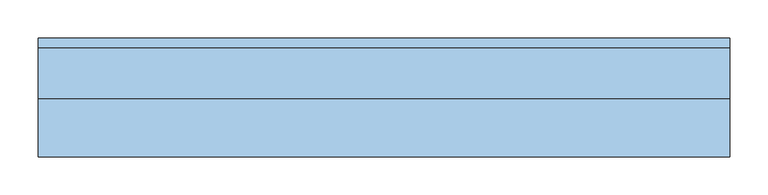
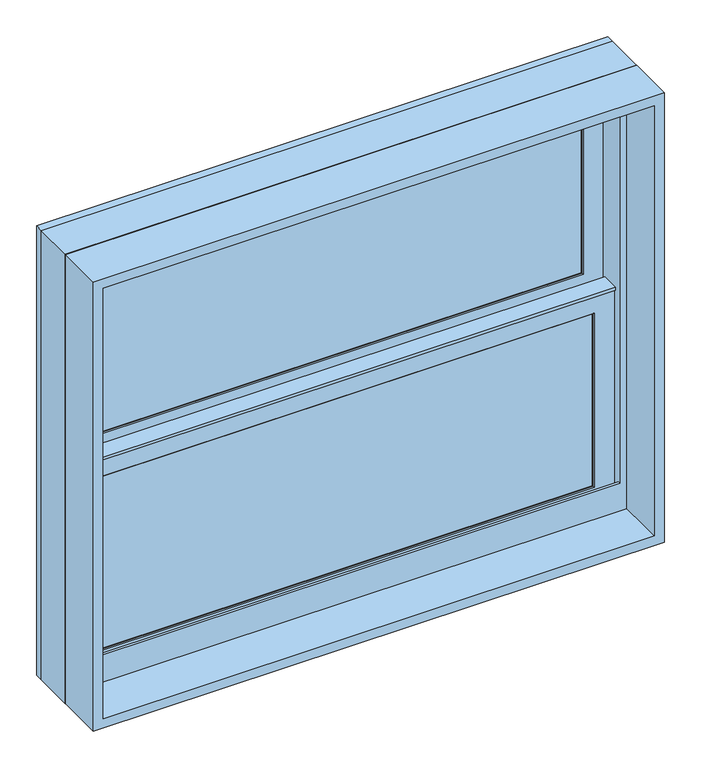
"""IFC4 building model written with IfcOpenShell, lengths in millimetres: window geometry, Window-Double_Hung-Marvin-Essential : ESDH3026."""

from ifc_helpers import new_model, si_unit, frame, origin, place, context, project, spatial, polyline, outline, extrude, faceted_brep, source, transform, mapped, element, save


def window_a7fb58c4(model_context):
    return source(origin(), model_context, "Body", "SolidModel", [
        extrude(outline(polyline([(140.7583333, 20.6375), (140.7583333, 15.875), (121.7083333, 15.875), (121.7083333, 20.6375), (140.7583333, 20.6375)])), frame((0.0, 0.0, 1746.25), z_axis=(0.0, 0.0, 1.0), x_axis=(1.0, 0.0, 0.0)), (0.0, 0.0, 1.0), 298.45),
        extrude(outline(polyline([(-121.7083333, 20.6375), (-121.7083333, 15.875), (-140.7583333, 15.875), (-140.7583333, 20.6375), (-121.7083333, 20.6375)])), frame((0.0, 0.0, 1746.25), z_axis=(0.0, 0.0, 1.0), x_axis=(1.0, 0.0, 0.0)), (0.0, 0.0, 1.0), 298.45),
        extrude(outline(polyline([(393.7, 20.6375), (393.7, 15.875), (-393.7, 15.875), (-393.7, 20.6375), (393.7, 20.6375)])), frame((0.0, 0.0, 1885.95), z_axis=(0.0, 0.0, 1.0), x_axis=(1.0, 0.0, 0.0)), (0.0, 0.0, 1.0), 19.05),
        extrude(outline(polyline([(-140.7583333, 46.83125), (-140.7583333, 51.59375), (-121.7083333, 51.59375), (-121.7083333, 46.83125), (-140.7583333, 46.83125)])), frame((0.0, 0.0, 2082.8), z_axis=(0.0, 0.0, 1.0), x_axis=(1.0, 0.0, 0.0)), (0.0, 0.0, 1.0), 298.45),
        extrude(outline(polyline([(121.7083333, 46.83125), (121.7083333, 51.59375), (140.7583333, 51.59375), (140.7583333, 46.83125), (121.7083333, 46.83125)])), frame((0.0, 0.0, 2082.8), z_axis=(0.0, 0.0, 1.0), x_axis=(1.0, 0.0, 0.0)), (0.0, 0.0, 1.0), 298.45),
        extrude(outline(polyline([(-393.7, 46.83125), (-393.7, 51.59375), (393.7, 51.59375), (393.7, 46.83125), (-393.7, 46.83125)])), frame((0.0, 0.0, 2222.5), z_axis=(0.0, 0.0, 1.0), x_axis=(1.0, 0.0, 0.0)), (0.0, 0.0, 1.0), 19.05),
        extrude(outline(polyline([(140.7583333, 20.6375), (121.7083333, 20.6375), (121.7083333, 25.4), (140.7583333, 25.4), (140.7583333, 20.6375)])), frame((0.0, 0.0, 1746.25), z_axis=(0.0, 0.0, 1.0), x_axis=(1.0, 0.0, 0.0)), (0.0, 0.0, 1.0), 298.45),
        extrude(outline(polyline([(-121.7083333, 20.6375), (-140.7583333, 20.6375), (-140.7583333, 25.4), (-121.7083333, 25.4), (-121.7083333, 20.6375)])), frame((0.0, 0.0, 1746.25), z_axis=(0.0, 0.0, 1.0), x_axis=(1.0, 0.0, 0.0)), (0.0, 0.0, 1.0), 298.45),
        extrude(outline(polyline([(393.7, 20.6375), (-393.7, 20.6375), (-393.7, 25.4), (393.7, 25.4), (393.7, 20.6375)])), frame((0.0, 0.0, 1885.95), z_axis=(0.0, 0.0, 1.0), x_axis=(1.0, 0.0, 0.0)), (0.0, 0.0, 1.0), 19.05),
        extrude(outline(polyline([(-140.7583333, 56.35625), (-121.7083333, 56.35625), (-121.7083333, 51.59375), (-140.7583333, 51.59375), (-140.7583333, 56.35625)])), frame((0.0, 0.0, 2082.8), z_axis=(0.0, 0.0, 1.0), x_axis=(1.0, 0.0, 0.0)), (0.0, 0.0, 1.0), 298.45),
        extrude(outline(polyline([(121.7083333, 56.35625), (140.7583333, 56.35625), (140.7583333, 51.59375), (121.7083333, 51.59375), (121.7083333, 56.35625)])), frame((0.0, 0.0, 2082.8), z_axis=(0.0, 0.0, 1.0), x_axis=(1.0, 0.0, 0.0)), (0.0, 0.0, 1.0), 298.45),
        extrude(outline(polyline([(-393.7, 56.35625), (393.7, 56.35625), (393.7, 51.59375), (-393.7, 51.59375), (-393.7, 56.35625)])), frame((0.0, 0.0, 2222.5), z_axis=(0.0, 0.0, 1.0), x_axis=(1.0, 0.0, 0.0)), (0.0, 0.0, 1.0), 19.05),
        faceted_brep([(-420.6875, 5.6780605, 2074.7351748), (-420.6875, 5.6780605, 2070.1), (420.6875, 5.6780605, 2070.1), (420.6875, 5.6780605, 2074.7351748), (-420.6875, 34.8118605, 2074.7351748), (420.6875, 34.8118605, 2074.7351748), (420.6875, 34.8118605, 2070.1), (-420.6875, 34.8118605, 2070.1), (-420.6875, 30.1625, 2070.1), (-420.6875, 30.1625, 1719.2625), (-420.6875, 8.9241104, 1719.2625), (-420.6875, 8.9241104, 2070.1), (420.6875, 8.9241104, 2070.1), (420.6875, 30.1625, 2070.1), (420.6875, 8.9241104, 1719.2625), (420.6875, 30.1625, 1719.2625), (-404.8034752, 11.90625, 2055.8034752), (-404.8034752, 30.1625, 2055.8034752), (404.8034752, 30.1625, 2055.8034752), (404.8034752, 11.90625, 2055.8034752), (-388.14375, 10.4662439, 2039.14375), (-388.14375, 11.90625, 2039.14375), (388.14375, 11.90625, 2039.14375), (388.14375, 10.4662439, 2039.14375), (389.6858834, 8.9241104, 2040.6858834), (-389.6858834, 8.9241104, 2040.6858834), (404.8034752, 30.1625, 1735.1465248), (404.8034752, 11.90625, 1735.1465248), (388.14375, 11.90625, 1751.80625), (388.14375, 10.4662439, 1751.80625), (389.6858834, 8.9241104, 1750.2641166), (-404.8034752, 30.1625, 1735.1465248), (-404.8034752, 11.90625, 1735.1465248), (-388.14375, 11.90625, 1751.80625), (-388.14375, 10.4662439, 1751.80625), (-389.6858834, 8.9241104, 1750.2641166)], [[[0, 1, 2, 3]], [[4, 5, 6, 7]], [[1, 0, 4, 7, 8, 9, 10, 11]], [[2, 1, 11, 12]], [[7, 6, 13, 8]], [[3, 2, 12, 14, 15, 13, 6, 5]], [[0, 3, 5, 4]], [[16, 17, 18, 19]], [[20, 21, 22, 23]], [[20, 23, 24, 25]], [[19, 18, 26, 27]], [[23, 22, 28, 29]], [[24, 23, 29, 30]], [[27, 26, 31, 32]], [[29, 28, 33, 34]], [[30, 29, 34, 35]], [[15, 14, 10, 9]], [[15, 9, 8, 13], [18, 17, 31, 26]], [[17, 16, 32, 31]], [[16, 19, 27, 32], [22, 21, 33, 28]], [[21, 20, 34, 33]], [[20, 25, 35, 34]], [[10, 14, 12, 11], [25, 24, 30, 35]]]),
        extrude(outline(polyline([(38.5955581, 2055.8125), (33.5778968, 2055.8125), (33.5778968, 2057.4), (39.9405976, 2057.4), (39.9405976, 2055.8125), (61.515625, 2055.8125), (47.6307501, 2052.4975159), (38.5955581, 2052.4975159), (38.5955581, 2055.8125)])), frame((-420.6875, 0.0, 0.0), z_axis=(1.0, 0.0, 0.0), x_axis=(0.0, 1.0, 0.0)), (0.0, 0.0, 1.0), 841.375),
        faceted_brep([(450.85, 0.0, 1689.1), (450.85, 0.0, 2438.4), (-450.85, 0.0, 2438.4), (-450.85, 0.0, 1689.1), (424.65625, 0.0, 1750.21875), (-424.65625, 0.0, 1750.21875), (-424.65625, 0.0, 2412.20625), (424.65625, 0.0, 2412.20625), (424.65625, 3.96875, 1689.1), (-424.65625, 3.96875, 1689.1), (-424.65625, 3.96875, 1750.21875), (424.65625, 3.96875, 1750.21875), (-450.85, 65.6828125, 1689.1), (-424.65625, 65.6828125, 1689.1), (424.65625, 65.6828125, 1689.1), (450.85, 65.6828125, 1689.1), (-450.85, 65.6828125, 2438.4), (450.85, 65.6828125, 2438.4), (424.65625, 65.6828125, 2412.20625), (-424.65625, 65.6828125, 2412.20625)], [[[0, 1, 2, 3], [4, 5, 6, 7]], [[8, 9, 10, 11]], [[5, 4, 11, 10]], [[0, 3, 12, 13, 9, 8, 14, 15]], [[13, 12, 16, 17, 15, 14, 18, 19]], [[13, 19, 6, 5, 10, 9]], [[7, 6, 19, 18]], [[18, 14, 8, 11, 4, 7]], [[1, 0, 15, 17]], [[2, 1, 17, 16]], [[3, 2, 16, 12]]]),
        faceted_brep([(424.65625, 30.1625, 2063.75), (423.06875, 30.1625, 2063.75), (423.06875, 30.1625, 1713.4544613), (424.65625, 30.1625, 1713.4544613), (-423.06875, 30.1625, 2063.75), (-424.65625, 30.1625, 2063.75), (-424.65625, 30.1625, 1713.4544613), (-423.06875, 30.1625, 1713.4544613), (423.06875, 63.5, 2063.75), (424.65625, 63.5, 2063.75), (424.65625, 63.5, 1706.9743077), (423.06875, 63.5, 1706.9743077), (-424.65625, 63.5, 2063.75), (-423.06875, 63.5, 2063.75), (-423.06875, 63.5, 1706.9743077), (-424.65625, 63.5, 1706.9743077), (435.9108932, 3.96875, 1718.5460105), (435.9108932, 3.96875, 1689.1), (435.9108932, 65.6828125, 1689.1), (435.9108932, 65.6828125, 1706.550012), (-435.9108932, 3.96875, 1689.1), (-435.9108932, 3.96875, 1718.5460105), (-435.9108932, 65.6828125, 1706.550012), (-435.9108932, 65.6828125, 1689.1), (435.9108932, 78.58125, 1704.0428097), (-435.9108932, 78.58125, 1704.0428097), (-433.8971252, 68.2348864, 1706.0539391), (-415.93135, 68.2348864, 1706.0539391), (-415.93135, 65.6828125, 1706.550012), (415.93135, 65.6828125, 1706.550012), (415.93135, 68.2348864, 1706.0539391), (433.8971252, 68.2348864, 1706.0539391), (-450.85, 65.6828125, 1689.1), (-450.85, 78.5948249, 1689.1), (450.85, 78.5948249, 1689.1), (450.85, 65.6828125, 1689.1), (-450.85, 78.58125, 2438.4), (450.85, 78.58125, 2438.4), (435.9108932, 78.58125, 2423.4608932), (-435.9108932, 78.58125, 2423.4608932), (-450.85, 65.6828125, 2438.4), (-433.8971252, 68.2348864, 2421.4471252), (433.8971252, 68.2348864, 2421.4471252), (415.93135, 68.2348864, 2403.48135), (-415.93135, 68.2348864, 2403.48135), (-415.93135, 65.6828125, 2403.48135), (415.93135, 65.6828125, 2403.48135), (450.85, 65.6828125, 2438.4)], [[[0, 1, 2, 3]], [[4, 5, 6, 7]], [[8, 9, 10, 11]], [[12, 13, 14, 15]], [[1, 8, 11, 2]], [[9, 0, 3, 10]], [[1, 0, 9, 8]], [[5, 4, 13, 12]], [[5, 12, 15, 6]], [[13, 4, 7, 14]], [[16, 17, 18, 19]], [[20, 21, 22, 23]], [[24, 25, 26, 27, 28, 22, 21, 16, 19, 29, 30, 31], [3, 2, 11, 10], [7, 6, 15, 14]], [[17, 16, 21, 20]], [[17, 20, 23, 32, 33, 34, 35, 18]], [[34, 33, 36, 37], [25, 24, 38, 39]], [[33, 32, 40, 36]], [[39, 41, 26, 25]], [[41, 42, 31, 30, 43, 44, 27, 26]], [[44, 45, 28, 27]], [[40, 32, 23, 22, 28, 45, 46, 29, 19, 18, 35, 47]], [[36, 40, 47, 37]], [[39, 38, 42, 41]], [[44, 43, 46, 45]], [[34, 37, 47, 35]], [[42, 38, 24, 31]], [[46, 43, 30, 29]]]),
        extrude(outline(polyline([(400.84375, 11.90625), (-400.84375, 11.90625), (-400.84375, 15.08125), (400.84375, 15.08125), (400.84375, 11.90625)])), frame((0.0, 0.0, 1739.10625), z_axis=(0.0, 0.0, 1.0), x_axis=(1.0, 0.0, 0.0)), (0.0, 0.0, 1.0), 312.7375),
        extrude(outline(polyline([(400.84375, 42.8625), (-400.84375, 42.8625), (-400.84375, 46.0375), (400.84375, 46.0375), (400.84375, 42.8625)])), frame((0.0, 0.0, 2075.65625), z_axis=(0.0, 0.0, 1.0), x_axis=(1.0, 0.0, 0.0)), (0.0, 0.0, 1.0), 312.7375),
        faceted_brep([(-388.14375, 31.194477, 2039.14375), (-389.6858834, 32.7366104, 2040.6858834), (389.6858834, 32.7366104, 2040.6858834), (388.14375, 31.194477, 2039.14375), (-388.14375, 30.1625, 2039.14375), (388.14375, 30.1625, 2039.14375), (-420.6875, 32.7366104, 2071.6875), (-420.6875, 30.1625, 2071.6875), (420.6875, 30.1625, 2071.6875), (420.6875, 32.7366104, 2071.6875), (389.6858834, 32.7366104, 1750.2641166), (388.14375, 31.194477, 1751.80625), (388.14375, 30.1625, 1751.80625), (420.6875, 30.1625, 1719.2625), (420.6875, 32.7366104, 1719.2625), (-389.6858834, 32.7366104, 1750.2641166), (-388.14375, 31.194477, 1751.80625), (-388.14375, 30.1625, 1751.80625), (-420.6875, 30.1625, 1719.2625), (-420.6875, 32.7366104, 1719.2625)], [[[0, 1, 2, 3]], [[4, 0, 3, 5]], [[6, 7, 8, 9]], [[3, 2, 10, 11]], [[5, 3, 11, 12]], [[9, 8, 13, 14]], [[11, 10, 15, 16]], [[12, 11, 16, 17]], [[14, 13, 18, 19]], [[9, 14, 19, 6], [1, 15, 10, 2]], [[16, 15, 1, 0]], [[17, 16, 0, 4]], [[7, 18, 13, 8], [5, 12, 17, 4]], [[19, 18, 7, 6]]]),
        faceted_brep([(-404.8034752, 42.8625, 2392.3534752), (-404.8034752, 61.11875, 2392.3534752), (404.8034752, 61.11875, 2392.3534752), (404.8034752, 42.8625, 2392.3534752), (-388.14375, 41.4224939, 2375.69375), (-388.14375, 42.8625, 2375.69375), (388.14375, 42.8625, 2375.69375), (388.14375, 41.4224939, 2375.69375), (-389.6858834, 39.8803604, 2377.2358834), (389.6858834, 39.8803604, 2377.2358834), (-420.6875, 61.11875, 2408.2375), (-420.6875, 39.8803604, 2408.2375), (420.6875, 39.8803604, 2408.2375), (420.6875, 61.11875, 2408.2375), (404.8034752, 61.11875, 2071.6965248), (404.8034752, 42.8625, 2071.6965248), (388.14375, 42.8625, 2088.35625), (388.14375, 41.4224939, 2088.35625), (389.6858834, 39.8803604, 2086.8141166), (420.6875, 39.8803604, 2055.8125), (420.6875, 61.11875, 2055.8125), (-404.8034752, 61.11875, 2071.6965248), (-404.8034752, 42.8625, 2071.6965248), (-388.14375, 42.8625, 2088.35625), (-388.14375, 41.4224939, 2088.35625), (-389.6858834, 39.8803604, 2086.8141166), (-420.6875, 39.8803604, 2055.8125), (-420.6875, 61.11875, 2055.8125)], [[[0, 1, 2, 3]], [[4, 5, 6, 7]], [[8, 4, 7, 9]], [[10, 11, 12, 13]], [[3, 2, 14, 15]], [[7, 6, 16, 17]], [[9, 7, 17, 18]], [[13, 12, 19, 20]], [[15, 14, 21, 22]], [[17, 16, 23, 24]], [[18, 17, 24, 25]], [[20, 19, 26, 27]], [[13, 20, 27, 10], [1, 21, 14, 2]], [[22, 21, 1, 0]], [[3, 15, 22, 0], [5, 23, 16, 6]], [[24, 23, 5, 4]], [[25, 24, 4, 8]], [[11, 26, 19, 12], [9, 18, 25, 8]], [[27, 26, 11, 10]]]),
        faceted_brep([(-420.6875, 61.11875, 2055.8125), (-420.6875, 63.6928604, 2055.8125), (420.6875, 63.6928604, 2055.8125), (420.6875, 61.11875, 2055.8125), (-388.14375, 62.150727, 2088.35625), (-388.14375, 61.11875, 2088.35625), (388.14375, 61.11875, 2088.35625), (388.14375, 62.150727, 2088.35625), (-389.6858834, 63.6928604, 2086.8141166), (389.6858834, 63.6928604, 2086.8141166), (420.6875, 63.6928604, 2408.2375), (420.6875, 61.11875, 2408.2375), (388.14375, 61.11875, 2375.69375), (388.14375, 62.150727, 2375.69375), (389.6858834, 63.6928604, 2377.2358834), (-420.6875, 63.6928604, 2408.2375), (-420.6875, 61.11875, 2408.2375), (-388.14375, 61.11875, 2375.69375), (-388.14375, 62.150727, 2375.69375), (-389.6858834, 63.6928604, 2377.2358834)], [[[0, 1, 2, 3]], [[4, 5, 6, 7]], [[8, 4, 7, 9]], [[3, 2, 10, 11]], [[7, 6, 12, 13]], [[9, 7, 13, 14]], [[11, 10, 15, 16]], [[13, 12, 17, 18]], [[14, 13, 18, 19]], [[16, 15, 1, 0]], [[3, 11, 16, 0], [5, 17, 12, 6]], [[18, 17, 5, 4]], [[19, 18, 4, 8]], [[1, 15, 10, 2], [9, 14, 19, 8]]]),
        extrude(outline(polyline([(400.84375, 26.19375), (-400.84375, 26.19375), (-400.84375, 30.1625), (400.84375, 30.1625), (400.84375, 26.19375)])), frame((0.0, 0.0, 1739.10625), z_axis=(0.0, 0.0, 1.0), x_axis=(1.0, 0.0, 0.0)), (0.0, 0.0, 1.0), 312.7375),
        extrude(outline(polyline([(400.84375, 57.15), (-400.84375, 57.15), (-400.84375, 61.11875), (400.84375, 61.11875), (400.84375, 57.15)])), frame((0.0, 0.0, 2075.65625), z_axis=(0.0, 0.0, 1.0), x_axis=(1.0, 0.0, 0.0)), (0.0, 0.0, 1.0), 312.7375),
        extrude(outline(polyline([(2438.4, 450.85), (2438.4, -450.85), (1689.1, -450.85), (1689.1, 450.85), (2438.4, 450.85)]), holes=[polyline([(2422.525, 434.975), (1704.975, 434.975), (1704.975, -434.975), (2422.525, -434.975), (2422.525, 434.975)])]), frame((0.0, -76.2, 0.0), z_axis=(0.0, 1.0, 0.0), x_axis=(0.0, 0.0, 1.0)), (0.0, 0.0, 1.0), 75.40625),
    ])


if __name__ == "__main__":
    model = new_model("IFC4")
    model_context = context("Model", 3, world=origin())
    ifc_project = project(units=[si_unit("LENGTHUNIT", "METRE", prefix="MILLI")], contexts=[model_context])
    site = spatial("IfcSite", under=ifc_project)
    building = spatial("IfcBuilding", under=site)
    placement = place(None, origin())
    window_shape = window_a7fb58c4(model_context)
    element("IfcWindow", 1, ObjectType="Window-Double_Hung-Marvin-Essential : ESDH3026", at=placement, inside=building, context=model_context, shape_type="MappedRepresentation", body=[
        mapped(window_shape, transform((0.0, 0.0, 0.0), x_axis=(1.0, 0.0, 0.0), y_axis=(0.0, 1.0, 0.0), z_axis=(0.0, 0.0, 1.0))),
    ])
    save(model, "model.ifc")

# Revit data of these elements
# Type "Window-Double_Hung-Marvin-Essential : ESDH3026"
#   Type Mark = "30"
#   Window Type = "Essential Double Hung"
#   Product data url = "https://bimobject.com/marvin-windows-and-doors/product/marvin-dhwau"
#   Product Guid = "c4a96547-874c-4385-91dc-a058adc19d98"
#   Frame = "All Ultrex"
#   Egress Window = "No"
#   URL = "www.marvin.com"
#   Model = "ESDH3026"
#   Manufacturer = "Marvin Windows and Doors"
#   Label Egress = ""
#   Glass Type = "IG Low E II with Argon"
#   Design Pressure = "DP50"
#   Description = "3630 DBHG"
#   Analytic Construction = "<None>"
#   Prairie Corner Width = 0' - 4"
#   Prairie Corner Height = 0' - 4"
#   Egress Width = 2' - 8 9/16"
#   Egress Height = 0' - 10 27/128"
#   Rough Width = 3' - 0"
#   Rough Height = 2' - 6"
#   Nominal Width = 3' - 0"
#   Nominal Height = 2' - 6"
#   Inset to Installation Flange [instance default] = 0' - 1"
#   Height = 2' - 5 1/2"
#   Egress Area = 2.30898 SF
#   Default Head Height = 8' - 0"
#   Width = 2' - 11 1/2"
#   Daylight Area = 4.80192 SF
#   DLO Width = 2' - 6 9/16"
#   DLO Height = 0' - 11 5/16"
#   Muntins Top Sash = yes
#   Lites Wide Top Sash = 3
#   Lites Wide Bottom Sash = 3
#   Lites High Top Sash = 2
#   Lites High Bottom Sash = 2
#   Lite Cut Prairie 9 = no
#   Lite Cut HV Grid = yes
#   Muntins Bottom Sash = yes
#   Label Visibility = no
#   Jamb Extension Visibility = yes
#   Edition number = 1
#   Interior Material = Ultrex-Marvin-Stonewhite
#   Glazing Material = Glass-Marvin-IG Low E II with Argon
#   Cladding Material = Ultrex-Marvin-Pebblegray
#   Wall Closure = (empty or 0)
#   Assembly Code = ""
# Element 1 (IfcWindow, "Window-Double_Hung-Marvin-Essential : ESDH3026")
#   Materials on its faces: "Ultrex-Marvin-Pebblegray", "Ultrex-Marvin-Stonewhite", "Glass-Marvin-IG Low E II with Argon"
# Materials
#   "Ultrex-Marvin-Stonewhite": class "Paint", colour RGB 250 251 245, transparency 0
#   "Glass-Marvin-IG Low E II with Argon": class "Glass", colour RGB 0 128 192, transparency 0.85
#   "Ultrex-Marvin-Pebblegray": class "Paint", colour RGB 189 185 173, transparency 0
